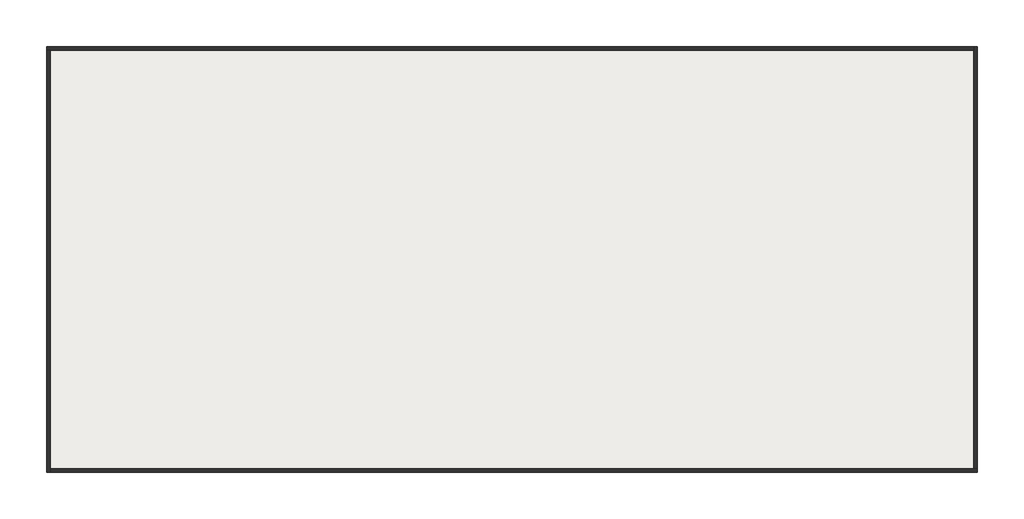
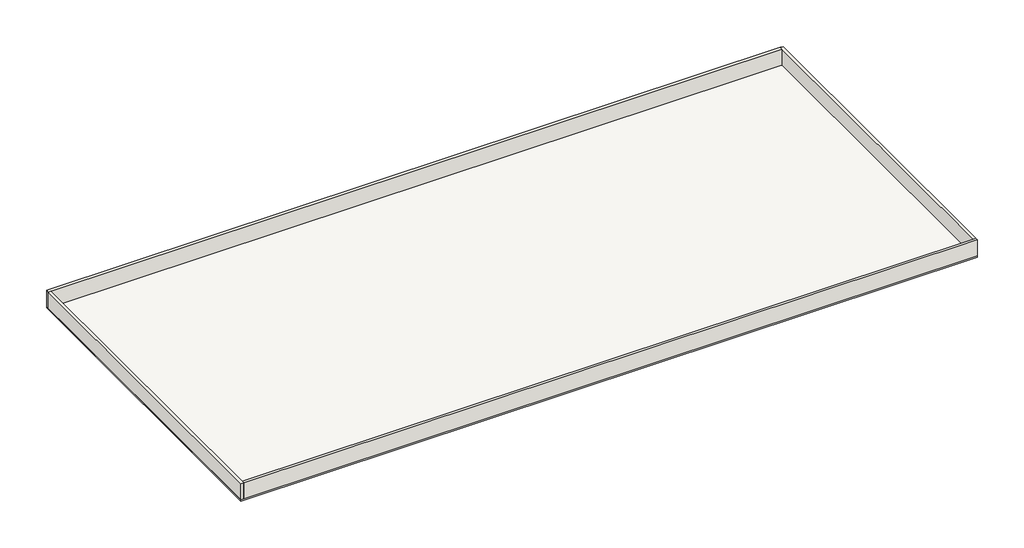
# One storey: 4 walls, 1 roof.
"""IFC4 building model written with IfcOpenShell, lengths in millimetres."""

import ifcopenshell
import ifcopenshell.guid

model = None  # the IFC model being written
_history = None  # IfcOwnerHistory: only IFC2X3 demands one
_inside = {}  # id of a spatial element -> (the spatial element, [elements in it])
_under = {}  # id of a project, library or spatial element -> (it, [spatial elements below it])
_declared = {}  # id of a project -> (the project, [libraries it declares])
_typed = {}  # id of a type object -> (the type object, [elements of that type])
_made_of = {}  # id of a material, layer set ... -> (it, [elements and type objects made of it])


def new_model(schema):
    """Start an empty IFC model of exactly this schema.

    Asked for "IFC4X3", IfcOpenShell would pick the latest addendum, in which some entities
    have other attributes; the version numbers below select the first issue.
    IFC2X3 requires an IfcOwnerHistory on every rooted entity: one is made here for all.
    """
    global model, _history
    if schema == "IFC4X3":
        model = ifcopenshell.file(schema_version=(4, 3, 0, 0))
    else:
        model = ifcopenshell.file(schema=schema)
    _inside.clear()
    _under.clear()
    _declared.clear()
    _typed.clear()
    _made_of.clear()
    _history = None
    if model.schema == "IFC2X3":
        org = make("IfcOrganization", Name="unknown")
        user = make(
            "IfcPersonAndOrganization",
            ThePerson=make("IfcPerson", FamilyName="unknown"),
            TheOrganization=org,
        )
        app = make(
            "IfcApplication",
            ApplicationDeveloper=org,
            Version="unknown",
            ApplicationFullName="unknown",
            ApplicationIdentifier="unknown",
        )
        _history = make(
            "IfcOwnerHistory",
            OwningUser=user,
            OwningApplication=app,
            ChangeAction="ADDED",
            CreationDate=0,
        )
    return model


def make(cls, **values):
    """One entity of the class cls with the attributes given. An attribute that is None is left unset."""
    return model.create_entity(
        cls, **{name: value for name, value in values.items() if value is not None}
    )


def rooted(cls, **values):
    """An entity with a GlobalId (a new one), such as an element, a storey or a relation."""
    return make(cls, GlobalId=ifcopenshell.guid.new(), OwnerHistory=_history, **values)


def si_unit(unit_type, name, prefix=None):
    """IfcSIUnit, for example si_unit("LENGTHUNIT", "METRE", prefix="MILLI")."""
    return make("IfcSIUnit", UnitType=unit_type, Prefix=prefix, Name=name)


def assignment(units):
    """IfcUnitAssignment: the units of a project."""
    return None if units is None else make("IfcUnitAssignment", Units=units)


def point(xyz):
    """IfcCartesianPoint."""
    return None if xyz is None else make("IfcCartesianPoint", Coordinates=xyz)


def direction(xyz):
    """IfcDirection."""
    return None if xyz is None else make("IfcDirection", DirectionRatios=xyz)


def frame(location, z_axis=None, x_axis=None):
    """IfcAxis2Placement3D, a coordinate frame: its origin and axes. An axis left out is left unset."""
    return make(
        "IfcAxis2Placement3D",
        Location=point(location),
        Axis=direction(z_axis),
        RefDirection=direction(x_axis),
    )


def origin():
    """The frame at (0, 0, 0) with its axes left unset."""
    return frame((0.0, 0.0, 0.0))


def place(relative_to, where):
    """IfcLocalPlacement: puts the frame where relative to a parent placement (None: the world)."""
    return make(
        "IfcLocalPlacement", PlacementRelTo=relative_to, RelativePlacement=where
    )


def context(
    kind, dimensions, precision=None, world=None, true_north=None, identifier=None
):
    """IfcGeometricRepresentationContext, for example the 3D "Model" context."""
    return make(
        "IfcGeometricRepresentationContext",
        ContextIdentifier=identifier,
        ContextType=kind,
        CoordinateSpaceDimension=dimensions,
        Precision=precision,
        WorldCoordinateSystem=world,
        TrueNorth=true_north,
    )


def project(units=None, contexts=None):
    """IfcProject with its units and contexts."""
    return rooted(
        "IfcProject",
        Name="project",
        RepresentationContexts=contexts,
        UnitsInContext=assignment(units),
    )


def spatial(cls, under=None, at=None, **own):
    """A site, building, storey or space (cls), placed at a placement, below another one or the project."""
    s = rooted(cls, ObjectPlacement=at, **own)
    if under is not None:
        _under.setdefault(under.id(), (under, []))[1].append(s)
    return s


def polyline(points):
    """IfcPolyline through the points."""
    return make("IfcPolyline", Points=[point(p) for p in points])


def outline(outer, holes=None, kind="AREA"):
    """IfcArbitraryClosedProfileDef: a profile drawn as a closed curve; with holes, ...WithVoids."""
    if holes is None:
        return make("IfcArbitraryClosedProfileDef", ProfileType=kind, OuterCurve=outer)
    return make(
        "IfcArbitraryProfileDefWithVoids",
        ProfileType=kind,
        OuterCurve=outer,
        InnerCurves=holes,
    )


def extrude(swept, where, along, depth):
    """IfcExtrudedAreaSolid: the profile swept, set in the frame where, extruded along a direction by depth."""
    return make(
        "IfcExtrudedAreaSolid",
        SweptArea=swept,
        Position=where,
        ExtrudedDirection=direction(along),
        Depth=depth,
    )


def faces_of(points, faces, orient=None, outer=None):
    """IfcFace entities. A face is a list of loops; a loop is a list of indices into points, from 0.

    orient and outer hold one flag for each loop. By default every Orientation is true, the
    first loop of a face is its IfcFaceOuterBound and the others are IfcFaceBound.
    """
    made = []
    for i, loops in enumerate(faces):
        bounds = []
        for j, loop in enumerate(loops):
            is_outer = j == 0 if outer is None else outer[i][j]
            bounds.append(
                make(
                    "IfcFaceOuterBound" if is_outer else "IfcFaceBound",
                    Bound=make("IfcPolyLoop", Polygon=[points[k] for k in loop]),
                    Orientation=True if orient is None else orient[i][j],
                )
            )
        made.append(make("IfcFace", Bounds=bounds))
    return made


def faceted_brep(points, faces, orient=None, outer=None, voids=None):
    """IfcFacetedBrep: a solid bounded by flat faces; with voids (closed shells), ...WithVoids."""
    shared = [point(p) for p in points]
    hull = make("IfcClosedShell", CfsFaces=faces_of(shared, faces, orient, outer))
    if voids is None:
        return make("IfcFacetedBrep", Outer=hull)
    return make(
        "IfcFacetedBrepWithVoids",
        Outer=hull,
        Voids=[
            make(cls, CfsFaces=faces_of(shared, fs, o, b)) for cls, fs, o, b in voids
        ],
    )


def shape(context_of_items, identifier, shape_type, items):
    """IfcShapeRepresentation: the items that make up one representation, for example the "Body"."""
    return make(
        "IfcShapeRepresentation",
        ContextOfItems=context_of_items,
        RepresentationIdentifier=identifier,
        RepresentationType=shape_type,
        Items=items,
    )


def made_of(thing, what):
    """Note that an element or type object is made of a material, layer set ...; save() writes the relation."""
    if what is not None:
        _made_of.setdefault(what.id(), (what, []))[1].append(thing)
    return thing


def element(
    cls,
    number,
    at=None,
    inside=None,
    cuts=None,
    type_object=None,
    material=None,
    context=None,
    identifier="Body",
    shape_type=None,
    held_by="IfcProductDefinitionShape",
    body=None,
    shapes=None,
    **own,
):
    """One element of the class cls, such as IfcWall. Its Tag is "e" and its number.

    at: its placement. inside: the storey or other place that contains it. cuts: it is an
    opening in that element (IfcRelVoidsElement). A single representation is given by context,
    identifier, shape_type and body (its items); several are given by shapes. held_by: the class
    of the entity that holds the representations. save() writes the other relations.
    """
    e = rooted(cls, Tag="e%d" % number, ObjectPlacement=at, **own)
    if body is not None:
        shapes = [shape(context, identifier, shape_type, body)]
    if shapes is not None:
        e.Representation = make(held_by, Representations=shapes)
    if inside is not None:
        _inside.setdefault(inside.id(), (inside, []))[1].append(e)
    if cuts is not None:
        rooted(
            "IfcRelVoidsElement", RelatingBuildingElement=cuts, RelatedOpeningElement=e
        )
    if type_object is not None:
        _typed.setdefault(type_object.id(), (type_object, []))[1].append(e)
    return made_of(e, material)


def aggregate(whole, parts):
    """IfcRelAggregates: a whole, such as a stair, and the parts it consists of."""
    return rooted("IfcRelAggregates", RelatingObject=whole, RelatedObjects=parts)


def save(model, path):
    """Write the relations noted so far, then the file.

    IfcRelAggregates (storeys below a building ...), IfcRelContainedInSpatialStructure (elements
    in a storey), IfcRelDefinesByType, IfcRelAssociatesMaterial and IfcRelDeclares: one each for
    every whole, place, type object, material and project.
    """
    for whole, parts in _under.values():
        aggregate(whole, parts)
    for where, things in _inside.values():
        rooted(
            "IfcRelContainedInSpatialStructure",
            RelatedElements=things,
            RelatingStructure=where,
        )
    for kind, things in _typed.values():
        rooted("IfcRelDefinesByType", RelatedObjects=things, RelatingType=kind)
    for what, things in _made_of.values():
        rooted("IfcRelAssociatesMaterial", RelatedObjects=things, RelatingMaterial=what)
    for by, libraries in _declared.values():
        rooted("IfcRelDeclares", RelatingContext=by, RelatedDefinitions=libraries)
    model.write(path)


model = new_model("IFC4")

# Units and contexts
model_context = context("Model", 3, world=origin())
ifc_project = project(units=[si_unit("LENGTHUNIT", "METRE", prefix="MILLI")], contexts=[model_context])

# Site, building, storey
site = spatial("IfcSite", under=ifc_project)
building = spatial("IfcBuilding", under=site)
storey = spatial("IfcBuildingStorey", under=building, Name="TOC", Elevation=7650.0)

# Roof
placement = place(None, origin())
element("IfcRoof", 1, ObjectType="H_RF_AMF_RC Roof Finish_WP_Insulation_Protection", at=placement, inside=storey, context=model_context, shape_type="SweptSolid", body=[
    extrude(outline(polyline([(53324.7, 24816.5208589), (53324.7, 216.5208589), (-475.3, 216.5208589), (-475.3, 24816.5208589), (53324.7, 24816.5208589)])), frame((0.0, 0.0, 7549.0), z_axis=(0.0, 0.0, 1.0), x_axis=(1.0, 0.0, 0.0)), (0.0, 0.0, 1.0), 101.0),
])

# Walls
element("IfcWall", 2, ObjectType="H_WA_AMW_RC Wall_T200 (No Finish)", at=placement, inside=storey, context=model_context, shape_type="Brep", body=[
    faceted_brep([(-475.3, 24616.5208589, 7650.0), (-275.3, 24616.5208589, 7650.0), (53124.7, 24616.5208589, 7650.0), (53124.7, 24616.5208589, 8900.0), (-275.3, 24616.5208589, 8900.0), (-475.3, 24616.5208589, 8900.0), (-475.3, 24816.5208589, 7650.0), (-475.3, 24816.5208589, 8900.0), (53124.7, 24816.5208589, 8900.0), (53124.7, 24816.5208589, 7650.0)], [[[0, 1, 2, 3, 4, 5]], [[6, 7, 8, 9]], [[2, 1, 0, 6, 9]], [[5, 4, 3, 8, 7]], [[0, 5, 7, 6]], [[3, 2, 9, 8]]]),
])
element("IfcWall", 3, ObjectType="H_WA_AMW_RC Wall_T200 (No Finish)", at=placement, inside=storey, context=model_context, shape_type="Brep", body=[
    faceted_brep([(-275.3, 216.5208589, 7650.0), (-275.3, 416.5208589, 7650.0), (-275.3, 24616.5208589, 7650.0), (-275.3, 24616.5208589, 8900.0), (-275.3, 416.5208589, 8900.0), (-275.3, 216.5208589, 8900.0), (-475.3, 216.5208589, 7650.0), (-475.3, 216.5208589, 8900.0), (-475.3, 24616.5208589, 8900.0), (-475.3, 24616.5208589, 7650.0)], [[[0, 1, 2, 3, 4, 5]], [[6, 7, 8, 9]], [[2, 1, 0, 6, 9]], [[5, 4, 3, 8, 7]], [[0, 5, 7, 6]], [[3, 2, 9, 8]]]),
])
element("IfcWall", 4, ObjectType="H_WA_AMW_RC Wall_T200 (No Finish)", at=placement, inside=storey, context=model_context, shape_type="Brep", body=[
    faceted_brep([(53324.7, 416.5208589, 7650.0), (53124.7, 416.5208589, 7650.0), (-275.3, 416.5208589, 7650.0), (-275.3, 416.5208589, 8900.0), (53124.7, 416.5208589, 8900.0), (53324.7, 416.5208589, 8900.0), (53324.7, 216.5208589, 7650.0), (53324.7, 216.5208589, 8900.0), (-275.3, 216.5208589, 8900.0), (-275.3, 216.5208589, 7650.0)], [[[0, 1, 2, 3, 4, 5]], [[6, 7, 8, 9]], [[2, 1, 0, 6, 9]], [[5, 4, 3, 8, 7]], [[0, 5, 7, 6]], [[3, 2, 9, 8]]]),
])
element("IfcWall", 5, ObjectType="H_WA_AMW_RC Wall_T200 (No Finish)", at=placement, inside=storey, context=model_context, shape_type="Brep", body=[
    faceted_brep([(53124.7, 24816.5208589, 7650.0), (53124.7, 24616.5208589, 7650.0), (53124.7, 416.5208589, 7650.0), (53124.7, 416.5208589, 8900.0), (53124.7, 24616.5208589, 8900.0), (53124.7, 24816.5208589, 8900.0), (53324.7, 24816.5208589, 7650.0), (53324.7, 24816.5208589, 8900.0), (53324.7, 416.5208589, 8900.0), (53324.7, 416.5208589, 7650.0)], [[[0, 1, 2, 3, 4, 5]], [[6, 7, 8, 9]], [[2, 1, 0, 6, 9]], [[5, 4, 3, 8, 7]], [[0, 5, 7, 6]], [[3, 2, 9, 8]]]),
])

save(model, "model.ifc")

# Revit data of these elements
# Type "H_RF_AMF_RC Roof Finish_WP_Insulation_Protection"
#   Layers, outside or top first: 0.050 m no material (function 4); 0.000 m no material (function 100); 0.050 m no material (function 3); 0.001 m no material (function 2)
# Type "H_WA_AMW_RC Wall_T200 (No Finish)"
#   Type Comments = ""
#   Layers, outside or top first: 0.000 m no material (function 100); 0.000 m no material (function 100); 0.200 m no material (function 1); 0.000 m no material (function 100); 0.000 m no material (function 100); 0.000 m no material (function 100)
# Element 1 (IfcRoof, "H_RF_AMF_RC Roof Finish_WP_Insulation_Protection")
#   built-in parameter 1001705 = 25.0984 (stored number, unit not read)
#   built-in parameter 1001701 = -0.331365 (stored number, unit not read)
#   built-in parameter 1001710 = 33615
#   Phase Created = New Construction
#   Materials on its faces: "Default Roof"
# Elements 2, 3, 4, 5 (IfcWall, "H_WA_AMW_RC Wall_T200 (No Finish)")
#   Top Offset = 0.000 m
#   Base Offset = 0.000 m
#   wall height = 1.250 m
#   Phase Created = New Construction
#   Base Constraint = TOC
#   Top Constraint = TOP
#   Materials on its faces: "Default Wall"
# Materials
#   "Default Roof": class "Miscellaneous", colour RGB 80 80 80, transparency 0
#   "Default Wall": class "Miscellaneous", colour RGB 80 80 80, transparency 0
